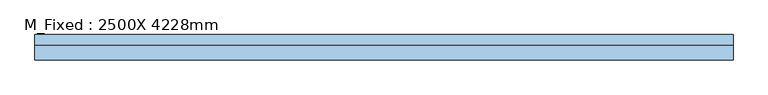
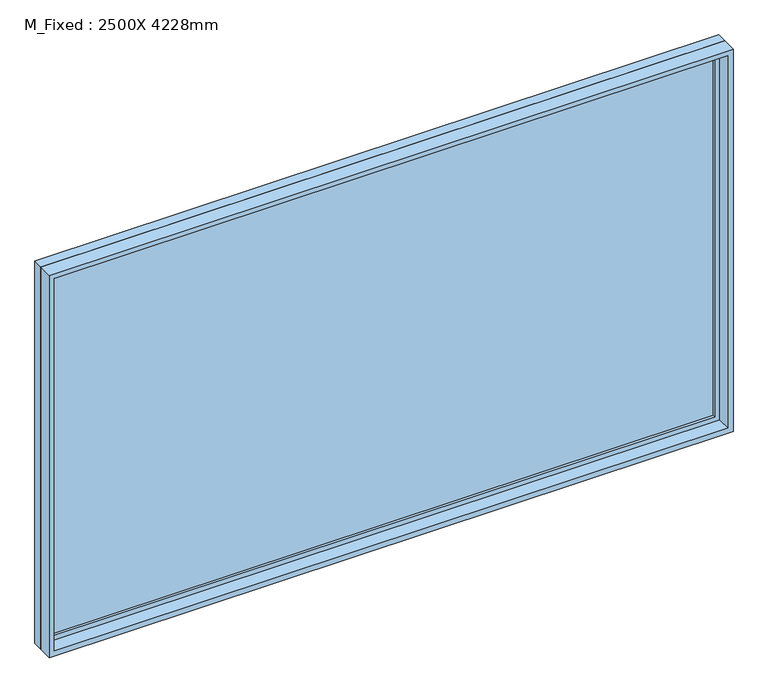
"""IFC4 building model written with IfcOpenShell, lengths in millimetres: window geometry, M_Fixed : 2500X 4228mm."""

import ifcopenshell
import ifcopenshell.guid

model = None  # the IFC model being written
_history = None  # IfcOwnerHistory: only IFC2X3 demands one
_inside = {}  # id of a spatial element -> (the spatial element, [elements in it])
_under = {}  # id of a project, library or spatial element -> (it, [spatial elements below it])
_declared = {}  # id of a project -> (the project, [libraries it declares])
_typed = {}  # id of a type object -> (the type object, [elements of that type])
_made_of = {}  # id of a material, layer set ... -> (it, [elements and type objects made of it])


def new_model(schema):
    """Start an empty IFC model of exactly this schema.

    Asked for "IFC4X3", IfcOpenShell would pick the latest addendum, in which some entities
    have other attributes; the version numbers below select the first issue.
    IFC2X3 requires an IfcOwnerHistory on every rooted entity: one is made here for all.
    """
    global model, _history
    if schema == "IFC4X3":
        model = ifcopenshell.file(schema_version=(4, 3, 0, 0))
    else:
        model = ifcopenshell.file(schema=schema)
    _inside.clear()
    _under.clear()
    _declared.clear()
    _typed.clear()
    _made_of.clear()
    _history = None
    if model.schema == "IFC2X3":
        org = make("IfcOrganization", Name="unknown")
        user = make(
            "IfcPersonAndOrganization",
            ThePerson=make("IfcPerson", FamilyName="unknown"),
            TheOrganization=org,
        )
        app = make(
            "IfcApplication",
            ApplicationDeveloper=org,
            Version="unknown",
            ApplicationFullName="unknown",
            ApplicationIdentifier="unknown",
        )
        _history = make(
            "IfcOwnerHistory",
            OwningUser=user,
            OwningApplication=app,
            ChangeAction="ADDED",
            CreationDate=0,
        )
    return model


def make(cls, **values):
    """One entity of the class cls with the attributes given. An attribute that is None is left unset."""
    return model.create_entity(
        cls, **{name: value for name, value in values.items() if value is not None}
    )


def rooted(cls, **values):
    """An entity with a GlobalId (a new one), such as an element, a storey or a relation."""
    return make(cls, GlobalId=ifcopenshell.guid.new(), OwnerHistory=_history, **values)


def si_unit(unit_type, name, prefix=None):
    """IfcSIUnit, for example si_unit("LENGTHUNIT", "METRE", prefix="MILLI")."""
    return make("IfcSIUnit", UnitType=unit_type, Prefix=prefix, Name=name)


def assignment(units):
    """IfcUnitAssignment: the units of a project."""
    return None if units is None else make("IfcUnitAssignment", Units=units)


def point(xyz):
    """IfcCartesianPoint."""
    return None if xyz is None else make("IfcCartesianPoint", Coordinates=xyz)


def direction(xyz):
    """IfcDirection."""
    return None if xyz is None else make("IfcDirection", DirectionRatios=xyz)


def frame(location, z_axis=None, x_axis=None):
    """IfcAxis2Placement3D, a coordinate frame: its origin and axes. An axis left out is left unset."""
    return make(
        "IfcAxis2Placement3D",
        Location=point(location),
        Axis=direction(z_axis),
        RefDirection=direction(x_axis),
    )


def origin():
    """The frame at (0, 0, 0) with its axes left unset."""
    return frame((0.0, 0.0, 0.0))


def place(relative_to, where):
    """IfcLocalPlacement: puts the frame where relative to a parent placement (None: the world)."""
    return make(
        "IfcLocalPlacement", PlacementRelTo=relative_to, RelativePlacement=where
    )


def context(
    kind, dimensions, precision=None, world=None, true_north=None, identifier=None
):
    """IfcGeometricRepresentationContext, for example the 3D "Model" context."""
    return make(
        "IfcGeometricRepresentationContext",
        ContextIdentifier=identifier,
        ContextType=kind,
        CoordinateSpaceDimension=dimensions,
        Precision=precision,
        WorldCoordinateSystem=world,
        TrueNorth=true_north,
    )


def project(units=None, contexts=None):
    """IfcProject with its units and contexts."""
    return rooted(
        "IfcProject",
        Name="project",
        RepresentationContexts=contexts,
        UnitsInContext=assignment(units),
    )


def spatial(cls, under=None, at=None, **own):
    """A site, building, storey or space (cls), placed at a placement, below another one or the project."""
    s = rooted(cls, ObjectPlacement=at, **own)
    if under is not None:
        _under.setdefault(under.id(), (under, []))[1].append(s)
    return s


def polyline(points):
    """IfcPolyline through the points."""
    return make("IfcPolyline", Points=[point(p) for p in points])


def outline(outer, holes=None, kind="AREA"):
    """IfcArbitraryClosedProfileDef: a profile drawn as a closed curve; with holes, ...WithVoids."""
    if holes is None:
        return make("IfcArbitraryClosedProfileDef", ProfileType=kind, OuterCurve=outer)
    return make(
        "IfcArbitraryProfileDefWithVoids",
        ProfileType=kind,
        OuterCurve=outer,
        InnerCurves=holes,
    )


def extrude(swept, where, along, depth):
    """IfcExtrudedAreaSolid: the profile swept, set in the frame where, extruded along a direction by depth."""
    return make(
        "IfcExtrudedAreaSolid",
        SweptArea=swept,
        Position=where,
        ExtrudedDirection=direction(along),
        Depth=depth,
    )


def shape(context_of_items, identifier, shape_type, items):
    """IfcShapeRepresentation: the items that make up one representation, for example the "Body"."""
    return make(
        "IfcShapeRepresentation",
        ContextOfItems=context_of_items,
        RepresentationIdentifier=identifier,
        RepresentationType=shape_type,
        Items=items,
    )


def source(mapping_origin, context_of_items, identifier, shape_type, items):
    """IfcRepresentationMap: a shape defined once, which mapped items show again and again."""
    return make(
        "IfcRepresentationMap",
        MappingOrigin=mapping_origin,
        MappedRepresentation=shape(context_of_items, identifier, shape_type, items),
    )


def transform(
    local_origin,
    x_axis=None,
    y_axis=None,
    z_axis=None,
    scale=None,
    scale2=None,
    scale3=None,
    uniform=True,
):
    """IfcCartesianTransformationOperator3D, or its non-uniform kind. x_axis, y_axis, z_axis: its Axis1, 2, 3."""
    if uniform:
        return make(
            "IfcCartesianTransformationOperator3D",
            Axis1=direction(x_axis),
            Axis2=direction(y_axis),
            LocalOrigin=point(local_origin),
            Scale=scale,
            Axis3=direction(z_axis),
        )
    return make(
        "IfcCartesianTransformationOperator3DnonUniform",
        Axis1=direction(x_axis),
        Axis2=direction(y_axis),
        LocalOrigin=point(local_origin),
        Scale=scale,
        Axis3=direction(z_axis),
        Scale2=scale2,
        Scale3=scale3,
    )


def mapped(mapping_source, mapping_target):
    """IfcMappedItem: shows the shape of a source again, moved by a transform."""
    return make(
        "IfcMappedItem", MappingSource=mapping_source, MappingTarget=mapping_target
    )


def made_of(thing, what):
    """Note that an element or type object is made of a material, layer set ...; save() writes the relation."""
    if what is not None:
        _made_of.setdefault(what.id(), (what, []))[1].append(thing)
    return thing


def element(
    cls,
    number,
    at=None,
    inside=None,
    cuts=None,
    type_object=None,
    material=None,
    context=None,
    identifier="Body",
    shape_type=None,
    held_by="IfcProductDefinitionShape",
    body=None,
    shapes=None,
    **own,
):
    """One element of the class cls, such as IfcWall. Its Tag is "e" and its number.

    at: its placement. inside: the storey or other place that contains it. cuts: it is an
    opening in that element (IfcRelVoidsElement). A single representation is given by context,
    identifier, shape_type and body (its items); several are given by shapes. held_by: the class
    of the entity that holds the representations. save() writes the other relations.
    """
    e = rooted(cls, Tag="e%d" % number, ObjectPlacement=at, **own)
    if body is not None:
        shapes = [shape(context, identifier, shape_type, body)]
    if shapes is not None:
        e.Representation = make(held_by, Representations=shapes)
    if inside is not None:
        _inside.setdefault(inside.id(), (inside, []))[1].append(e)
    if cuts is not None:
        rooted(
            "IfcRelVoidsElement", RelatingBuildingElement=cuts, RelatedOpeningElement=e
        )
    if type_object is not None:
        _typed.setdefault(type_object.id(), (type_object, []))[1].append(e)
    return made_of(e, material)


def aggregate(whole, parts):
    """IfcRelAggregates: a whole, such as a stair, and the parts it consists of."""
    return rooted("IfcRelAggregates", RelatingObject=whole, RelatedObjects=parts)


def save(model, path):
    """Write the relations noted so far, then the file.

    IfcRelAggregates (storeys below a building ...), IfcRelContainedInSpatialStructure (elements
    in a storey), IfcRelDefinesByType, IfcRelAssociatesMaterial and IfcRelDeclares: one each for
    every whole, place, type object, material and project.
    """
    for whole, parts in _under.values():
        aggregate(whole, parts)
    for where, things in _inside.values():
        rooted(
            "IfcRelContainedInSpatialStructure",
            RelatedElements=things,
            RelatingStructure=where,
        )
    for kind, things in _typed.values():
        rooted("IfcRelDefinesByType", RelatedObjects=things, RelatingType=kind)
    for what, things in _made_of.values():
        rooted("IfcRelAssociatesMaterial", RelatedObjects=things, RelatingMaterial=what)
    for by, libraries in _declared.values():
        rooted("IfcRelDeclares", RelatingContext=by, RelatedDefinitions=libraries)
    model.write(path)


def m_fixed_2500x_4228mm_fd5e51e7(model_context):
    return source(origin(), model_context, "Body", "SweptSolid", [
        extrude(outline(polyline([(-2050.8, 54.2), (2050.8, 54.2), (2050.8, 42.2), (-2050.8, 42.2), (-2050.8, 54.2)])), frame((0.0, 0.0, 368.0), z_axis=(0.0, 0.0, 1.0), x_axis=(1.0, 0.0, 0.0)), (0.0, 0.0, 1.0), 2374.0),
        extrude(outline(polyline([(2786.0, -2094.8), (324.0, -2094.8), (324.0, 2094.8), (2786.0, 2094.8), (2786.0, -2094.8)]), holes=[polyline([(2742.0, -2050.8), (2742.0, 2050.8), (368.0, 2050.8), (368.0, -2050.8), (2742.0, -2050.8)])]), frame((0.0, 26.2, 0.0), z_axis=(0.0, 1.0, 0.0), x_axis=(0.0, 0.0, 1.0)), (0.0, 0.0, 1.0), 44.0),
        extrude(outline(polyline([(2805.0, -2113.8), (305.0, -2113.8), (305.0, 2113.8), (2805.0, 2113.8), (2805.0, -2113.8)]), holes=[polyline([(2786.0, -2094.8), (2786.0, 2094.8), (324.0, 2094.8), (324.0, -2094.8), (2786.0, -2094.8)])]), frame((0.0, 26.2, 0.0), z_axis=(0.0, 1.0, 0.0), x_axis=(0.0, 0.0, 1.0)), (0.0, 0.0, 1.0), 63.0),
        extrude(outline(polyline([(2805.0, -2113.8), (305.0, -2113.8), (305.0, 2113.8), (2805.0, 2113.8), (2805.0, -2113.8)]), holes=[polyline([(2773.0, -2081.8), (2773.0, 2081.8), (337.0, 2081.8), (337.0, -2081.8), (2773.0, -2081.8)])]), frame((0.0, -63.2, 0.0), z_axis=(0.0, 1.0, 0.0), x_axis=(0.0, 0.0, 1.0)), (0.0, 0.0, 1.0), 89.4),
    ])


if __name__ == "__main__":
    model = new_model("IFC4")
    model_context = context("Model", 3, world=origin())
    ifc_project = project(units=[si_unit("LENGTHUNIT", "METRE", prefix="MILLI")], contexts=[model_context])
    site = spatial("IfcSite", under=ifc_project)
    building = spatial("IfcBuilding", under=site)
    placement = place(None, origin())
    m_fixed_2500x_4228mm_shape = m_fixed_2500x_4228mm_fd5e51e7(model_context)
    element("IfcWindow", 1, ObjectType="M_Fixed : 2500X 4228mm", at=placement, inside=building, context=model_context, shape_type="MappedRepresentation", body=[
        mapped(m_fixed_2500x_4228mm_shape, transform((0.0, 0.0, 0.0), x_axis=(1.0, 0.0, 0.0), y_axis=(0.0, 1.0, 0.0), z_axis=(0.0, 0.0, 1.0))),
    ])
    save(model, "model.ifc")

# Revit data of these elements
# Type "M_Fixed : 2500X 4228mm"
#   Type Mark = "25"
#   Height = 2500 mm
#   Default Sill Height = 305 mm
#   Width = 4227.6 mm
#   Window Inset = 19 mm
#   Frame Exterior Material = Sash
#   Frame Interior Material = Sash
#   Glass Pane Material = Glass
#   Sash = Sash
#   Wall Closure = (empty or 0)
# Element 1 (IfcWindow, "M_Fixed : 2500X 4228mm")
#   Materials on its faces: "Sash", "Glass"
# Materials
#   "Sash": class "Wood", colour RGB 136 99 55, transparency 0
#   "Glass": class "Glass", colour RGB 0 128 192, transparency 0.9, Description = "Soda Lime Glass", Cost = 0
